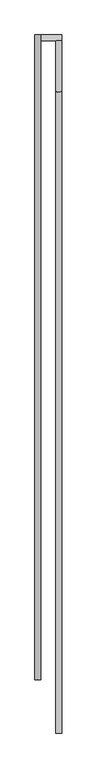
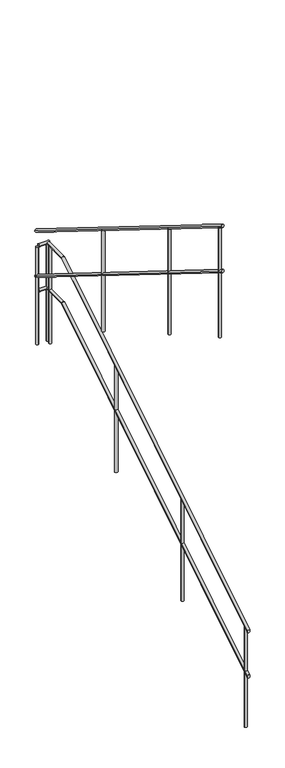
"""IFC4 building model written with IfcOpenShell, lengths in millimetres: railing geometry."""

from ifc_helpers import new_model, si_unit, point, frame, frame_2d, origin, place, context, project, spatial, circle_curve, ellipse_curve, trimmed, segment, composite_curve, outline, extrude, source, transform, mapped, element, save
from ifc_brep_helpers import plane_surface, cylinder_surface, advanced_brep


def railing_1ac2519f(model_context):
    return source(origin(), model_context, "Body", "SolidModel", [
        advanced_brep(
        [(11545.1052251, 14699.5208589, 456.3396197), (11515.1052251, 14699.5208589, 456.3396197), (11545.1052251, 18329.5208589, 2547.0), (11515.1052251, 18329.5208589, 2547.0), (11545.1052251, 18063.8019306, 2547.0), (11515.1052251, 18063.8019306, 2547.0)],
        [
            (0, 1, ellipse_curve(frame((11530.1052251, 14699.5208589, 456.3396197), z_axis=(0.0, -1.0, 0.0), x_axis=(0.0, 0.0, -1.0)), 17.6603803, 15.0)),
            (1, 0, ellipse_curve(frame((11530.1052251, 14699.5208589, 456.3396197), z_axis=(0.0, -1.0, 0.0), x_axis=(0.0, 0.0, -1.0)), 17.6603803, 15.0)),
            (2, 3, circle_curve(frame((11530.1052251, 18329.5208589, 2547.0), z_axis=(0.0, 1.0, 0.0), x_axis=(-1.0, 0.0, 0.0)), 15.0)),
            (3, 2, circle_curve(frame((11530.1052251, 18329.5208589, 2547.0), z_axis=(0.0, 1.0, 0.0), x_axis=(-1.0, 0.0, 0.0)), 15.0)),
            (0, 4),
            (4, 5, ellipse_curve(frame((11530.1052251, 18063.8019306, 2547.0), z_axis=(0.0, -0.9616025257983003, -0.2744459552959912), x_axis=(0.0, 0.2744459552959914, -0.9616025257983002)), 15.5989607, 15.0)),
            (5, 1),
            (5, 4, ellipse_curve(frame((11530.1052251, 18063.8019306, 2547.0), z_axis=(0.0, -0.9616025257983003, -0.2744459552959912), x_axis=(0.0, 0.2744459552959914, -0.9616025257983002)), 15.5989607, 15.0)),
            (4, 2),
            (3, 5),
        ],
        [
            plane_surface(frame((11530.1052251, 14699.5208589, 474.0), z_axis=(0.0, -1.0, 0.0), x_axis=(0.0, 0.0, 1.0))),
            plane_surface(frame((11530.1052251, 18329.5208589, 2562.0), z_axis=(0.0, 1.0, 0.0), x_axis=(0.0, 0.0, 1.0))),
            cylinder_surface(frame((11530.1052251, 14707.4380966, 461.2596175), z_axis=(0.0, -0.8493588352433417, -0.5278158476155052), x_axis=(-1.0, 0.0, 0.0)), 15.0),
            cylinder_surface(frame((11530.1052251, 18059.5208589, 2547.0), z_axis=(0.0, -1.0, 0.0), x_axis=(-1.0, 0.0, 0.0)), 15.0),
        ],
        [
            (0, [[1, 2]]),
            (1, [[3, 4]]),
            (2, [[-1, 5, 6, 7]]),
            (2, [[-2, -7, 8, -5]]),
            (3, [[-6, 9, -4, 10]]),
            (3, [[-8, -10, -3, -9]]),
        ],
    ),
        advanced_brep(
        [(11545.1052251, 18359.5208589, 2547.0), (11545.1052251, 18329.5208589, 2547.0), (11435.1052251, 18359.5208589, 2547.0), (11435.1052251, 18329.5208589, 2547.0)],
        [
            (0, 1, circle_curve(frame((11545.1052251, 18344.5208589, 2547.0), z_axis=(1.0, 0.0, 0.0), x_axis=(0.0, -1.0, 0.0)), 15.0)),
            (1, 0, circle_curve(frame((11545.1052251, 18344.5208589, 2547.0), z_axis=(1.0, 0.0, 0.0), x_axis=(0.0, -1.0, 0.0)), 15.0)),
            (2, 3, circle_curve(frame((11435.1052251, 18344.5208589, 2547.0), z_axis=(-1.0, 0.0, 0.0), x_axis=(0.0, -1.0, 0.0)), 15.0)),
            (3, 2, circle_curve(frame((11435.1052251, 18344.5208589, 2547.0), z_axis=(-1.0, 0.0, 0.0), x_axis=(0.0, -1.0, 0.0)), 15.0)),
            (0, 2),
            (3, 1),
        ],
        [
            plane_surface(frame((11545.1052251, 18344.5208589, 2562.0), z_axis=(1.0, 0.0, 0.0), x_axis=(0.0, -1.0, 0.0))),
            plane_surface(frame((11435.1052251, 18344.5208589, 2562.0), z_axis=(-1.0, 0.0, 0.0), x_axis=(0.0, -1.0, 0.0))),
            cylinder_surface(frame((11545.1052251, 18344.5208589, 2547.0), z_axis=(1.0, 0.0, 0.0), x_axis=(0.0, -1.0, 0.0)), 15.0),
        ],
        [
            (0, [[1, 2]]),
            (1, [[3, 4]]),
            (2, [[-1, 5, -4, 6]]),
            (2, [[-2, -6, -3, -5]]),
        ],
    ),
        advanced_brep(
        [(11405.1052251, 18359.5208589, 2705.9110483), (11435.1052251, 18359.5208589, 2705.9110483), (11405.1052251, 14979.5208589, 4806.3396197), (11435.1052251, 14979.5208589, 4806.3396197)],
        [
            (0, 1, ellipse_curve(frame((11420.1052251, 18359.5208589, 2705.9110483), z_axis=(0.0, 1.0, 0.0), x_axis=(0.0, 0.0, -1.0)), 17.6603803, 15.0)),
            (1, 0, ellipse_curve(frame((11420.1052251, 18359.5208589, 2705.9110483), z_axis=(0.0, 1.0, 0.0), x_axis=(0.0, 0.0, -1.0)), 17.6603803, 15.0)),
            (2, 3, ellipse_curve(frame((11420.1052251, 14979.5208589, 4806.3396197), z_axis=(0.0, -1.0, 0.0), x_axis=(0.0, 0.0, -1.0)), 17.6603803, 15.0)),
            (3, 2, ellipse_curve(frame((11420.1052251, 14979.5208589, 4806.3396197), z_axis=(0.0, -1.0, 0.0), x_axis=(0.0, 0.0, -1.0)), 17.6603803, 15.0)),
            (0, 2),
            (3, 1),
        ],
        [
            plane_surface(frame((11420.1052251, 18359.5208589, 2723.5714286), z_axis=(0.0, 1.0, 0.0), x_axis=(0.0, 0.0, -1.0))),
            plane_surface(frame((11420.1052251, 14979.5208589, 4824.0), z_axis=(0.0, -1.0, 0.0), x_axis=(0.0, 0.0, -1.0))),
            cylinder_surface(frame((11420.1052251, 18351.6036212, 2710.831046), z_axis=(0.0, 0.8493588352433417, -0.5278158476155052), x_axis=(1.0, 0.0, 0.0)), 15.0),
        ],
        [
            (0, [[1, 2]]),
            (1, [[3, 4]]),
            (2, [[-1, 5, -4, 6]]),
            (2, [[-2, -6, -3, -5]]),
        ],
    ),
        advanced_brep(
        [(11545.1052251, 14699.5208589, 956.3396197), (11515.1052251, 14699.5208589, 956.3396197), (11545.1052251, 18063.8019306, 3047.0), (11515.1052251, 18063.8019306, 3047.0), (11545.1052251, 18329.5208589, 3047.0), (11515.1052251, 18329.5208589, 3047.0)],
        [
            (0, 1, ellipse_curve(frame((11530.1052251, 14699.5208589, 956.3396197), z_axis=(0.0, -1.0, 0.0), x_axis=(0.0, 0.0, -1.0)), 17.6603803, 15.0)),
            (1, 0, ellipse_curve(frame((11530.1052251, 14699.5208589, 956.3396197), z_axis=(0.0, -1.0, 0.0), x_axis=(0.0, 0.0, -1.0)), 17.6603803, 15.0)),
            (0, 2),
            (2, 3, ellipse_curve(frame((11530.1052251, 18063.8019306, 3047.0), z_axis=(0.0, -0.9616025257983003, -0.2744459552959912), x_axis=(0.0, 0.2744459552959914, -0.9616025257983002)), 15.5989607, 15.0)),
            (3, 1),
            (3, 2, ellipse_curve(frame((11530.1052251, 18063.8019306, 3047.0), z_axis=(0.0, -0.9616025257983003, -0.2744459552959912), x_axis=(0.0, 0.2744459552959914, -0.9616025257983002)), 15.5989607, 15.0)),
            (4, 5, circle_curve(frame((11530.1052251, 18329.5208589, 3047.0), z_axis=(0.0, 1.0, 0.0), x_axis=(-1.0, 0.0, 0.0)), 15.0)),
            (5, 4, circle_curve(frame((11530.1052251, 18329.5208589, 3047.0), z_axis=(0.0, 1.0, 0.0), x_axis=(-1.0, 0.0, 0.0)), 15.0)),
            (2, 4),
            (5, 3),
        ],
        [
            plane_surface(frame((11530.1052251, 14699.5208589, 974.0), z_axis=(0.0, -1.0, 0.0), x_axis=(0.0, 0.0, 1.0))),
            cylinder_surface(frame((11530.1052251, 14707.4380966, 961.2596175), z_axis=(0.0, -0.8493588352433417, -0.5278158476155052), x_axis=(-1.0, 0.0, 0.0)), 15.0),
            plane_surface(frame((11530.1052251, 18329.5208589, 3062.0), z_axis=(0.0, 1.0, 0.0), x_axis=(0.0, 0.0, 1.0))),
            cylinder_surface(frame((11530.1052251, 18059.5208589, 3047.0), z_axis=(0.0, -1.0, 0.0), x_axis=(-1.0, 0.0, 0.0)), 15.0),
        ],
        [
            (0, [[1, 2]]),
            (1, [[-1, 3, 4, 5]]),
            (1, [[-2, -5, 6, -3]]),
            (2, [[7, 8]]),
            (3, [[-4, 9, -8, 10]]),
            (3, [[-6, -10, -7, -9]]),
        ],
    ),
        advanced_brep(
        [(11545.1052251, 18359.5208589, 3047.0), (11545.1052251, 18329.5208589, 3047.0), (11435.1052251, 18359.5208589, 3047.0), (11435.1052251, 18329.5208589, 3047.0)],
        [
            (0, 1, circle_curve(frame((11545.1052251, 18344.5208589, 3047.0), z_axis=(1.0, 0.0, 0.0), x_axis=(0.0, -1.0, 0.0)), 15.0)),
            (1, 0, circle_curve(frame((11545.1052251, 18344.5208589, 3047.0), z_axis=(1.0, 0.0, 0.0), x_axis=(0.0, -1.0, 0.0)), 15.0)),
            (2, 3, circle_curve(frame((11435.1052251, 18344.5208589, 3047.0), z_axis=(-1.0, 0.0, 0.0), x_axis=(0.0, -1.0, 0.0)), 15.0)),
            (3, 2, circle_curve(frame((11435.1052251, 18344.5208589, 3047.0), z_axis=(-1.0, 0.0, 0.0), x_axis=(0.0, -1.0, 0.0)), 15.0)),
            (0, 2),
            (3, 1),
        ],
        [
            plane_surface(frame((11545.1052251, 18344.5208589, 3062.0), z_axis=(1.0, 0.0, 0.0), x_axis=(0.0, -1.0, 0.0))),
            plane_surface(frame((11435.1052251, 18344.5208589, 3062.0), z_axis=(-1.0, 0.0, 0.0), x_axis=(0.0, -1.0, 0.0))),
            cylinder_surface(frame((11545.1052251, 18344.5208589, 3047.0), z_axis=(1.0, 0.0, 0.0), x_axis=(0.0, -1.0, 0.0)), 15.0),
        ],
        [
            (0, [[1, 2]]),
            (1, [[3, 4]]),
            (2, [[-1, 5, -4, 6]]),
            (2, [[-2, -6, -3, -5]]),
        ],
    ),
        advanced_brep(
        [(11405.1052251, 18359.5208589, 3205.9110483), (11435.1052251, 18359.5208589, 3205.9110483), (11405.1052251, 14979.5208589, 5306.3396197), (11435.1052251, 14979.5208589, 5306.3396197)],
        [
            (0, 1, ellipse_curve(frame((11420.1052251, 18359.5208589, 3205.9110483), z_axis=(0.0, 1.0, 0.0), x_axis=(0.0, 0.0, -1.0)), 17.6603803, 15.0)),
            (1, 0, ellipse_curve(frame((11420.1052251, 18359.5208589, 3205.9110483), z_axis=(0.0, 1.0, 0.0), x_axis=(0.0, 0.0, -1.0)), 17.6603803, 15.0)),
            (2, 3, ellipse_curve(frame((11420.1052251, 14979.5208589, 5306.3396197), z_axis=(0.0, -1.0, 0.0), x_axis=(0.0, 0.0, -1.0)), 17.6603803, 15.0)),
            (3, 2, ellipse_curve(frame((11420.1052251, 14979.5208589, 5306.3396197), z_axis=(0.0, -1.0, 0.0), x_axis=(0.0, 0.0, -1.0)), 17.6603803, 15.0)),
            (0, 2),
            (3, 1),
        ],
        [
            plane_surface(frame((11420.1052251, 18359.5208589, 3223.5714286), z_axis=(0.0, 1.0, 0.0), x_axis=(0.0, 0.0, -1.0))),
            plane_surface(frame((11420.1052251, 14979.5208589, 5324.0), z_axis=(0.0, -1.0, 0.0), x_axis=(0.0, 0.0, -1.0))),
            cylinder_surface(frame((11420.1052251, 18351.6036212, 3210.831046), z_axis=(0.0, 0.8493588352433417, -0.5278158476155052), x_axis=(1.0, 0.0, 0.0)), 15.0),
        ],
        [
            (0, [[1, 2]]),
            (1, [[3, 4]]),
            (2, [[-1, 5, -4, 6]]),
            (2, [[-2, -6, -3, -5]]),
        ],
    ),
        extrude(outline(composite_curve([segment(trimmed(circle_curve(frame_2d((11420.1052251, 15944.5208589)), 15.0), [point((11435.1052251, 15944.5208589))], [point((11405.1052251, 15944.5208589))], False, "CARTESIAN"), True, "CONTINUOUS"), segment(trimmed(circle_curve(frame_2d((11420.1052251, 15944.5208589)), 15.0), [point((11405.1052251, 15944.5208589))], [point((11435.1052251, 15944.5208589))], False, "CARTESIAN"), True, "CONTINUOUS")], self_intersect=False)), frame((0.0, 0.0, 3528.0), z_axis=(0.0, 0.0, 1.0), x_axis=(1.0, 0.0, 0.0)), (0.0, 0.0, 1.0), 1166.3214286),
        extrude(outline(composite_curve([segment(trimmed(circle_curve(frame_2d((11420.1052251, 17144.5208589)), 15.0), [point((11435.1052251, 17144.5208589))], [point((11405.1052251, 17144.5208589))], False, "CARTESIAN"), True, "CONTINUOUS"), segment(trimmed(circle_curve(frame_2d((11420.1052251, 17144.5208589)), 15.0), [point((11405.1052251, 17144.5208589))], [point((11435.1052251, 17144.5208589))], False, "CARTESIAN"), True, "CONTINUOUS")], self_intersect=False)), frame((0.0, 0.0, 2832.0), z_axis=(0.0, 0.0, 1.0), x_axis=(1.0, 0.0, 0.0)), (0.0, 0.0, 1.0), 1116.6071429),
        extrude(outline(composite_curve([segment(trimmed(circle_curve(frame_2d((11530.1052251, 18299.5208589)), 15.0), [point((11515.1052251, 18299.5208589))], [point((11545.1052251, 18299.5208589))], False, "CARTESIAN"), True, "CONTINUOUS"), segment(trimmed(circle_curve(frame_2d((11530.1052251, 18299.5208589)), 15.0), [point((11545.1052251, 18299.5208589))], [point((11515.1052251, 18299.5208589))], False, "CARTESIAN"), True, "CONTINUOUS")], self_intersect=False)), frame((0.0, 0.0, 1962.0), z_axis=(0.0, 0.0, 1.0), x_axis=(1.0, 0.0, 0.0)), (0.0, 0.0, 1.0), 1070.0),
        extrude(outline(composite_curve([segment(trimmed(circle_curve(frame_2d((11530.1052251, 17099.5208589)), 15.0), [point((11515.1052251, 17099.5208589))], [point((11545.1052251, 17099.5208589))], False, "CARTESIAN"), True, "CONTINUOUS"), segment(trimmed(circle_curve(frame_2d((11530.1052251, 17099.5208589)), 15.0), [point((11545.1052251, 17099.5208589))], [point((11515.1052251, 17099.5208589))], False, "CARTESIAN"), True, "CONTINUOUS")], self_intersect=False)), frame((0.0, 0.0, 1266.0), z_axis=(0.0, 0.0, 1.0), x_axis=(1.0, 0.0, 0.0)), (0.0, 0.0, 1.0), 1169.4285714),
        extrude(outline(composite_curve([segment(trimmed(circle_curve(frame_2d((11530.1052251, 15899.5208589)), 15.0), [point((11515.1052251, 15899.5208589))], [point((11545.1052251, 15899.5208589))], False, "CARTESIAN"), True, "CONTINUOUS"), segment(trimmed(circle_curve(frame_2d((11530.1052251, 15899.5208589)), 15.0), [point((11545.1052251, 15899.5208589))], [point((11515.1052251, 15899.5208589))], False, "CARTESIAN"), True, "CONTINUOUS")], self_intersect=False)), frame((0.0, 0.0, 570.0), z_axis=(0.0, 0.0, 1.0), x_axis=(1.0, 0.0, 0.0)), (0.0, 0.0, 1.0), 1119.7142857),
        extrude(outline(composite_curve([segment(trimmed(circle_curve(frame_2d((11420.1052251, 18344.5208589)), 15.0), [point((11420.1052251, 18329.5208589))], [point((11420.1052251, 18359.5208589))], False, "CARTESIAN"), True, "CONTINUOUS"), segment(trimmed(circle_curve(frame_2d((11420.1052251, 18344.5208589)), 15.0), [point((11420.1052251, 18359.5208589))], [point((11420.1052251, 18329.5208589))], False, "CARTESIAN"), True, "CONTINUOUS")], self_intersect=False)), frame((0.0, 0.0, 1962.0), z_axis=(0.0, 0.0, 1.0), x_axis=(1.0, 0.0, 0.0)), (0.0, 0.0, 1.0), 1070.0),
        extrude(outline(composite_curve([segment(trimmed(circle_curve(frame_2d((11530.1052251, 18344.5208589)), 15.0), [point((11515.1052251, 18344.5208589))], [point((11545.1052251, 18344.5208589))], False, "CARTESIAN"), True, "CONTINUOUS"), segment(trimmed(circle_curve(frame_2d((11530.1052251, 18344.5208589)), 15.0), [point((11545.1052251, 18344.5208589))], [point((11515.1052251, 18344.5208589))], False, "CARTESIAN"), True, "CONTINUOUS")], self_intersect=False)), frame((0.0, 0.0, 1962.0), z_axis=(0.0, 0.0, 1.0), x_axis=(1.0, 0.0, 0.0)), (0.0, 0.0, 1.0), 1070.0),
        extrude(outline(composite_curve([segment(trimmed(circle_curve(frame_2d((11420.1052251, 15029.5208589)), 15.0), [point((11435.1052251, 15029.5208589))], [point((11405.1052251, 15029.5208589))], False, "CARTESIAN"), True, "CONTINUOUS"), segment(trimmed(circle_curve(frame_2d((11420.1052251, 15029.5208589)), 15.0), [point((11405.1052251, 15029.5208589))], [point((11435.1052251, 15029.5208589))], False, "CARTESIAN"), True, "CONTINUOUS")], self_intersect=False)), frame((0.0, 0.0, 4050.0), z_axis=(0.0, 0.0, 1.0), x_axis=(1.0, 0.0, 0.0)), (0.0, 0.0, 1.0), 1212.9285714),
        extrude(outline(composite_curve([segment(trimmed(circle_curve(frame_2d((11530.1052251, 14749.5208589)), 15.0), [point((11515.1052251, 14749.5208589))], [point((11545.1052251, 14749.5208589))], False, "CARTESIAN"), True, "CONTINUOUS"), segment(trimmed(circle_curve(frame_2d((11530.1052251, 14749.5208589)), 15.0), [point((11545.1052251, 14749.5208589))], [point((11515.1052251, 14749.5208589))], False, "CARTESIAN"), True, "CONTINUOUS")], self_intersect=False)), frame((0.0, 0.0, -126.0), z_axis=(0.0, 0.0, 1.0), x_axis=(1.0, 0.0, 0.0)), (0.0, 0.0, 1.0), 1101.0714286),
    ])


if __name__ == "__main__":
    model = new_model("IFC4")
    model_context = context("Model", 3, world=origin())
    ifc_project = project(units=[si_unit("LENGTHUNIT", "METRE", prefix="MILLI")], contexts=[model_context])
    site = spatial("IfcSite", under=ifc_project)
    building = spatial("IfcBuilding", under=site)
    placement = place(None, origin())
    railing_shape = railing_1ac2519f(model_context)
    element("IfcRailing", 1, at=placement, inside=building, context=model_context, shape_type="MappedRepresentation", body=[
        mapped(railing_shape, transform((0.0, 0.0, 0.0), x_axis=(1.0, 0.0, 0.0), y_axis=(0.0, 1.0, 0.0), z_axis=(0.0, 0.0, 1.0))),
    ])
    save(model, "model.ifc")
